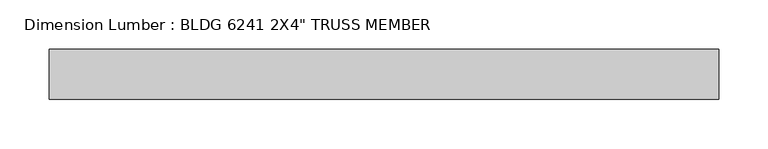
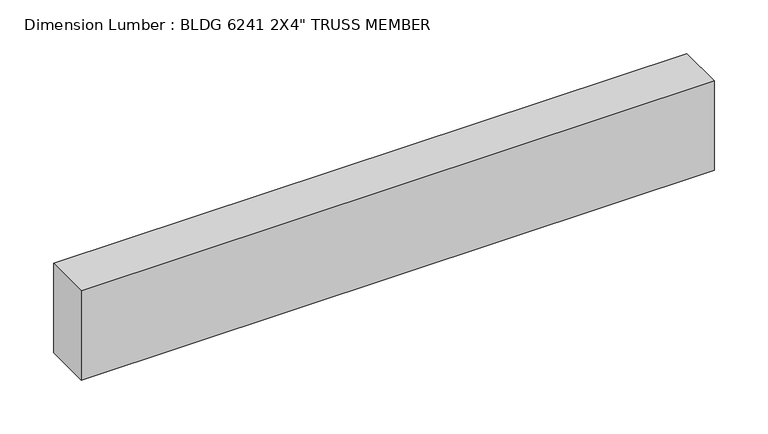
"""IFC4 building model written with IfcOpenShell, lengths in millimetres: beam geometry."""

from ifc_helpers import new_model, si_unit, frame, origin, place, context, project, spatial, polyline, outline, extrude, source, transform, mapped, element, save


def beam_9afb64f6(model_context):
    return source(origin(), model_context, "Body", "SweptSolid", [
        extrude(outline(polyline([(365.3019367, 25.4), (365.3019367, -25.4), (-314.5019367, -25.4), (-314.5019367, 25.4), (365.3019367, 25.4)])), frame((0.0, 0.0, -50.8), z_axis=(0.0, 0.0, 1.0), x_axis=(1.0, 0.0, 0.0)), (0.0, 0.0, 1.0), 101.6),
    ])


if __name__ == "__main__":
    model = new_model("IFC4")
    model_context = context("Model", 3, world=origin())
    ifc_project = project(units=[si_unit("LENGTHUNIT", "METRE", prefix="MILLI")], contexts=[model_context])
    site = spatial("IfcSite", under=ifc_project)
    building = spatial("IfcBuilding", under=site)
    placement = place(None, origin())
    beam_shape = beam_9afb64f6(model_context)
    element("IfcBeam", 1, ObjectType="Dimension Lumber : BLDG 6241 2X4\" TRUSS MEMBER", at=placement, inside=building, context=model_context, shape_type="MappedRepresentation", body=[
        mapped(beam_shape, transform((0.0, 0.0, 0.0), x_axis=(1.0, 0.0, 0.0), y_axis=(0.0, 1.0, 0.0), z_axis=(0.0, 0.0, 1.0))),
    ])
    save(model, "model.ifc")

# Revit data of these elements
# Type "Dimension Lumber : BLDG 6241 2X4\" TRUSS MEMBER"
#   Assembly Code = "B10"
#   A = 0.273472 SF
#   Length [instance default] = 5' - 0"
#   b = 0' - 2"
#   d = 0' - 4"
#   Structural Material [instance default] = Softwood, Lumber
# Element 1 (IfcBeam, "Dimension Lumber : BLDG 6241 2X4\" TRUSS MEMBER")
#   Materials on its faces: "Softwood, Lumber"
# Materials
#   "Softwood, Lumber": class "Wood", colour RGB 223 192 134, transparency 0, Description = "Pinus Echinata", Cost = 0
